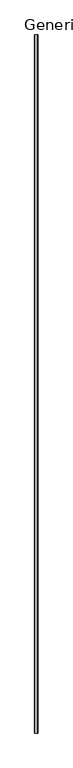
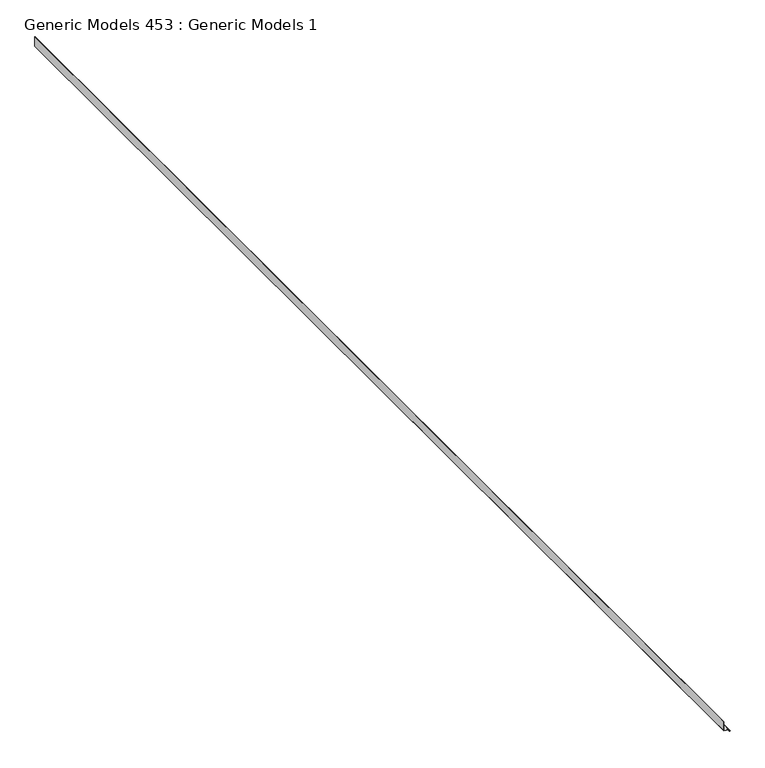
"""IFC4 building model written with IfcOpenShell, lengths in millimetres: proxy geometry, Generic Models 453 : Generic Models 1."""

from ifc_helpers import new_model, si_unit, point, frame, frame_2d, origin, place, context, project, spatial, polyline, circle_curve, trimmed, segment, composite_curve, outline, extrude, source, transform, mapped, element, save


def generic_models_453_generic_models_1_94991b40(model_context):
    return source(origin(), model_context, "Body", "SweptSolid", [
        extrude(outline(composite_curve([segment(polyline([(129128.7798285, 1639.7527532), (129126.0332953, 1671.1457713), (129118.1755711, 1679.0034954)]), True, "CONTINUOUS"), segment(trimmed(circle_curve(frame_2d((129117.0530391, 1677.8809634)), 1.5875), [point((129118.1755711, 1679.0034954))], [point((129115.9305071, 1679.0034954))], True, "CARTESIAN"), True, "CONTINUOUS"), segment(polyline([(129115.9305071, 1679.0034954), (129115.3692411, 1678.4422294)]), True, "CONTINUOUS"), segment(trimmed(circle_curve(frame_2d((129116.4917731, 1677.3196974)), 1.5875), [point((129115.3692411, 1678.4422294))], [point((129115.3692411, 1676.1971654))], True, "CARTESIAN"), True, "CONTINUOUS"), segment(polyline([(129115.3692411, 1676.1971654), (129123.2269652, 1668.3394413), (129122.6656992, 1667.7781753), (129114.8079751, 1675.6358994)]), True, "CONTINUOUS"), segment(trimmed(circle_curve(frame_2d((129116.4917731, 1677.3196974)), 2.38125), [point((129114.8079751, 1675.6358994))], [point((129114.8079751, 1679.0034954))], False, "CARTESIAN"), True, "CONTINUOUS"), segment(polyline([(129114.8079751, 1679.0034954), (129115.3692411, 1679.5647615)]), True, "CONTINUOUS"), segment(trimmed(circle_curve(frame_2d((129117.0530391, 1677.8809634)), 2.38125), [point((129115.3692411, 1679.5647615))], [point((129118.7368372, 1679.5647615))], False, "CARTESIAN"), True, "CONTINUOUS"), segment(polyline([(129118.7368372, 1679.5647615), (129126.7988454, 1671.5027532), (129129.5071663, 1640.5465032), (129192.2798285, 1640.5465032), (129192.2798285, 1639.7527532), (129128.7798285, 1639.7527532)]), True, "CONTINUOUS")], self_intersect=False)), frame((0.0, 306.6963299, 0.0), z_axis=(0.0, 1.0, 0.0), x_axis=(0.0, 0.0, 1.0)), (0.0, 0.0, 1.0), 7886.7),
    ])


if __name__ == "__main__":
    model = new_model("IFC4")
    model_context = context("Model", 3, world=origin())
    ifc_project = project(units=[si_unit("LENGTHUNIT", "METRE", prefix="MILLI")], contexts=[model_context])
    site = spatial("IfcSite", under=ifc_project)
    building = spatial("IfcBuilding", under=site)
    placement = place(None, origin())
    generic_models_453_generic_models_1_shape = generic_models_453_generic_models_1_94991b40(model_context)
    element("IfcBuildingElementProxy", 1, Name="Generic Models 453 : Generic Models 1", ObjectType="Generic Models 453 : Generic Models 1", at=placement, inside=building, context=model_context, shape_type="MappedRepresentation", body=[
        mapped(generic_models_453_generic_models_1_shape, transform((0.0, 0.0, 0.0), x_axis=(1.0, 0.0, 0.0), y_axis=(0.0, 1.0, 0.0), z_axis=(0.0, 0.0, 1.0))),
    ])
    save(model, "model.ifc")

# Revit data of these elements
# Element 1 (IfcBuildingElementProxy, "Generic Models 453 : Generic Models 1")
#   Materials on its faces: "_CONT. 16 GA. COPPER DRIP FLASHING"
# Materials
#   "_CONT. 16 GA. COPPER DRIP FLASHING": class "Metal", colour RGB 199 199 199, transparency 0, Description = "Structural steel 50ksi", Cost = 0
